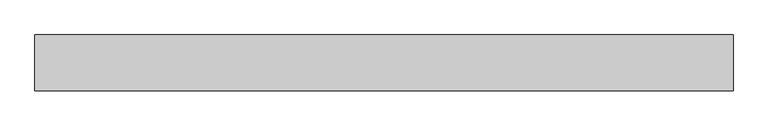
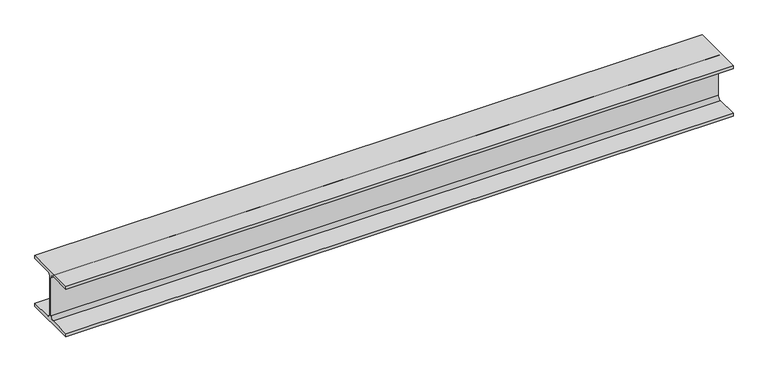
"""IFC4 building model written with IfcOpenShell, lengths in millimetres: beam geometry, 0912_Steel Framing_H-KSD3502 : H_SB_ASB_H-200x200x8x12."""

from ifc_helpers import new_model, si_unit, point, frame, frame_2d, origin, place, context, project, spatial, polyline, circle_curve, trimmed, segment, composite_curve, outline, extrude, source, transform, mapped, element, save


def beam_1d2e41cb(model_context):
    return source(origin(), model_context, "Body", "SweptSolid", [
        extrude(outline(composite_curve([segment(polyline([(100.0, -88.0), (100.0, -100.0), (-100.0, -100.0), (-100.0, -88.0), (-17.0, -88.0)]), True, "CONTINUOUS"), segment(trimmed(circle_curve(frame_2d((-17.0, -75.0)), 13.0), [point((-17.0, -88.0))], [point((-4.0, -75.0))], True, "CARTESIAN"), True, "CONTINUOUS"), segment(polyline([(-4.0, -75.0), (-4.0, 75.0)]), True, "CONTINUOUS"), segment(trimmed(circle_curve(frame_2d((-17.0, 75.0)), 13.0), [point((-4.0, 75.0))], [point((-17.0, 88.0))], True, "CARTESIAN"), True, "CONTINUOUS"), segment(polyline([(-17.0, 88.0), (-100.0, 88.0), (-100.0, 100.0), (100.0, 100.0), (100.0, 88.0), (17.0, 88.0)]), True, "CONTINUOUS"), segment(trimmed(circle_curve(frame_2d((17.0, 75.0)), 13.0), [point((17.0, 88.0))], [point((4.0, 75.0))], True, "CARTESIAN"), True, "CONTINUOUS"), segment(polyline([(4.0, 75.0), (4.0, -75.0)]), True, "CONTINUOUS"), segment(trimmed(circle_curve(frame_2d((17.0, -75.0)), 13.0), [point((4.0, -75.0))], [point((17.0, -88.0))], True, "CARTESIAN"), True, "CONTINUOUS"), segment(polyline([(17.0, -88.0), (100.0, -88.0)]), True, "CONTINUOUS")], self_intersect=False)), frame((-1270.5762137, 0.0, 0.0), z_axis=(1.0, 0.0, 0.0), x_axis=(0.0, 1.0, 0.0)), (0.0, 0.0, 1.0), 2490.6760125),
    ])


if __name__ == "__main__":
    model = new_model("IFC4")
    model_context = context("Model", 3, world=origin())
    ifc_project = project(units=[si_unit("LENGTHUNIT", "METRE", prefix="MILLI")], contexts=[model_context])
    site = spatial("IfcSite", under=ifc_project)
    building = spatial("IfcBuilding", under=site)
    placement = place(None, origin())
    beam_shape = beam_1d2e41cb(model_context)
    element("IfcBeam", 1, ObjectType="0912_Steel Framing_H-KSD3502 : H_SB_ASB_H-200x200x8x12", at=placement, inside=building, context=model_context, shape_type="MappedRepresentation", body=[
        mapped(beam_shape, transform((0.0, 0.0, 0.0), x_axis=(1.0, 0.0, 0.0), y_axis=(0.0, 1.0, 0.0), z_axis=(0.0, 0.0, 1.0))),
    ])
    save(model, "model.ifc")

# Revit data of these elements
# Type "0912_Steel Framing_H-KSD3502 : H_SB_ASB_H-200x200x8x12"
#   H_WM Code_1 = "S01AA002-00001 | Main Steel Structure Fabrication Work | Shelter/Building | Medium Steel - Standard (90KG/M>Weight≥30KG/M) | Material: (   )"
#   H_WM Code_2 = "S03AA028-00001 | Main Steel Structure Erection Work | Shelter/Building | Medium Steel (90KG/M>Weight≥30KG/M) | Material: (   )"
#   H_WM Code_3 = "S01AA010-00001 | Main Steel Structure Fabrication Work | Shelter/Building | Steel Painting/Coating | for Non-Fireproofed Steel Surface, Surface Preparation, Primer, Second & Final Coat | Material: (   )"
#   H_Q'ty Cal Type Tag = "SB-Q2"
#   Width = 20.0 cm
#   Web Thickness = 0.8 cm
#   Web Fillet = 1.3 cm
#   Warping Constant = 141000.0 cm⁶
#   W = 0
#   Torsional Moment of Inertia = 26.2485 cm⁴
#   Section Area = 63.53 cm²
#   Plastic Modulus weak axis = 244.0 cm³
#   Plastic Modulus strong axis = 525.0 cm³
#   Perimeter = 1.16 m²/m
#   Nominal Weight = 49.90 kgf/m
#   Moment of Inertia weak axis = 1600.00 cm⁴
#   Moment of Inertia strong axis = 4720.00 cm⁴
#   Height = 20.0 cm
#   Flange Thickness = 1.2 cm
#   Elastic Modulus weak axis = 160.0 cm³
#   Elastic Modulus strong axis = 472.0 cm³
#   Centroid Vertical = 10.0 cm
#   Centroid Horizontal = 10.0 cm
#   Ix = 47200000
#   Length [instance default] = 1.5240 m
#   Zx = 525000
#   b = 0.2000 m
#   h = 0.2000 m
#   r = 0.0130 m
#   s = 0.0080 m
#   t = 0.0120 m
#   A = 0.006353 m²
#   Structural Material [instance default] = Steel, 45-345
#   Assembly Code = ""
# Element 1 (IfcBeam, "0912_Steel Framing_H-KSD3502 : H_SB_ASB_H-200x200x8x12")
#   Structural Material = none
# Materials
#   "Steel, 45-345": class "Metal", colour RGB 189 187 185, transparency 0, Description = "Steel 345 MPa", Cost = 0
